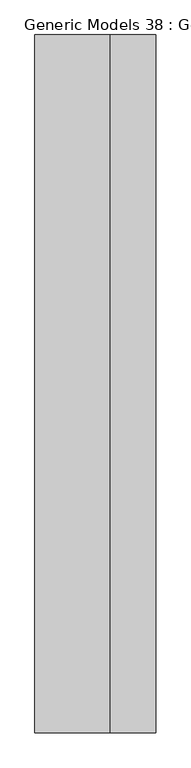
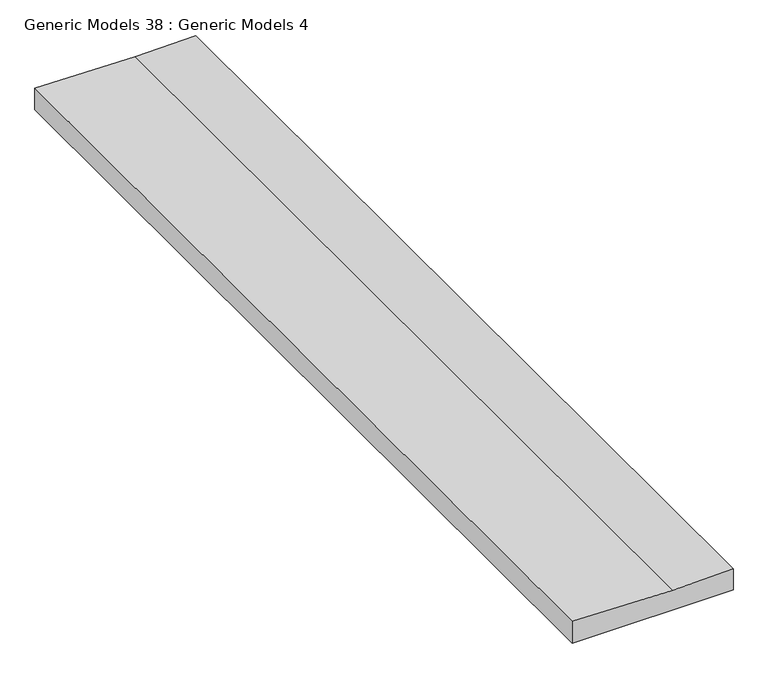
"""IFC4 building model written with IfcOpenShell, lengths in millimetres: proxy geometry, Generic Models 38 : Generic Models 4."""

from ifc_helpers import new_model, si_unit, frame, origin, place, context, project, spatial, polyline, outline, extrude, source, transform, mapped, element, save


def generic_models_38_generic_models_4_0a67166e(model_context):
    return source(origin(), model_context, "Body", "SweptSolid", [
        extrude(outline(polyline([(126790.196, 7337.1724037), (126790.196, 8153.9657764), (126901.9317168, 8153.9657764), (126895.5332396, 7846.8388704), (126906.151291, 7337.1724037), (126790.196, 7337.1724037)])), frame((0.0, 7054.2769662, 0.0), z_axis=(0.0, 1.0, 0.0), x_axis=(0.0, 0.0, 1.0)), (0.0, 0.0, 1.0), 4724.4),
    ])


if __name__ == "__main__":
    model = new_model("IFC4")
    model_context = context("Model", 3, world=origin())
    ifc_project = project(units=[si_unit("LENGTHUNIT", "METRE", prefix="MILLI")], contexts=[model_context])
    site = spatial("IfcSite", under=ifc_project)
    building = spatial("IfcBuilding", under=site)
    placement = place(None, origin())
    generic_models_38_generic_models_4_shape = generic_models_38_generic_models_4_0a67166e(model_context)
    element("IfcBuildingElementProxy", 1, Name="Generic Models 38 : Generic Models 4", ObjectType="Generic Models 38 : Generic Models 4", at=placement, inside=building, context=model_context, shape_type="MappedRepresentation", body=[
        mapped(generic_models_38_generic_models_4_shape, transform((0.0, 0.0, 0.0), x_axis=(1.0, 0.0, 0.0), y_axis=(0.0, 1.0, 0.0), z_axis=(0.0, 0.0, 1.0))),
    ])
    save(model, "model.ifc")

# Revit data of these elements
# Element 1 (IfcBuildingElementProxy, "Generic Models 38 : Generic Models 4")
#   Materials on its faces: "_EPS INSULATION - TAPER TO DRAINS (X\" MIN DEPTH - (X) MIN. R-FACTOR)"
# Materials
#   "_EPS INSULATION - TAPER TO DRAINS (X\" MIN DEPTH - (X) MIN. R-FACTOR)": class "Generic", colour RGB 245 226 173, transparency 0, Cost = 0
